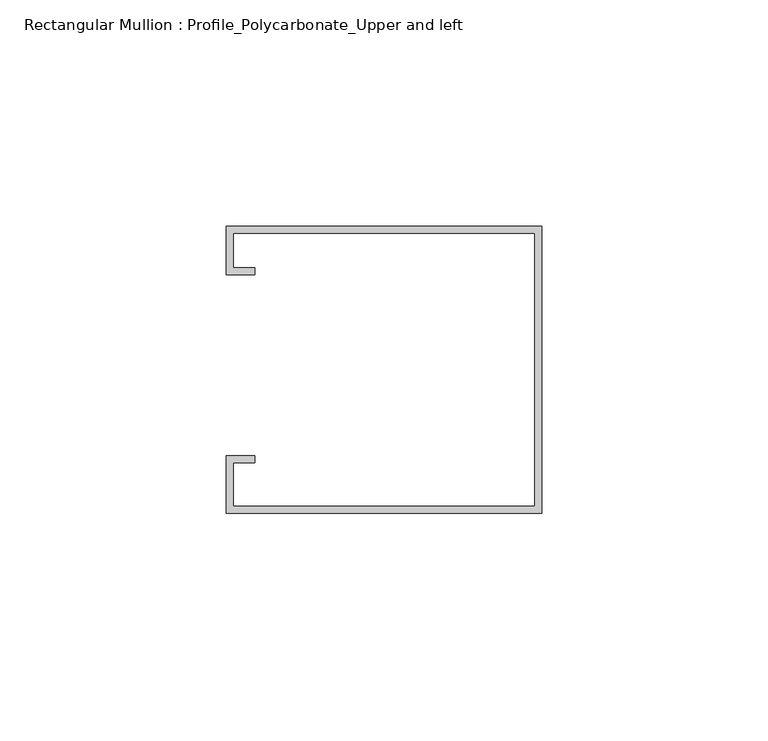
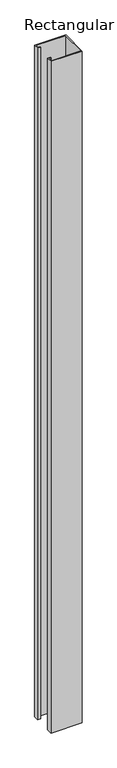
"""IFC4 building model written with IfcOpenShell, lengths in millimetres: member geometry, Rectangular Mullion : Profile_Polycarbonate_Upper and left."""

from ifc_helpers import new_model, si_unit, frame, origin, place, context, project, spatial, polyline, outline, extrude, source, transform, mapped, element, save


def rectangular_mullion_profile_polycarbonate_upper_and_left_256955de(model_context):
    return source(origin(), model_context, "Body", "SweptSolid", [
        extrude(outline(polyline([(0.0, -32.7), (-69.85, -32.7), (-69.85, -20.0), (-63.5, -20.0), (-63.5, -21.5875), (-68.2625, -21.5875), (-68.2625, -31.1125), (-1.5875, -31.1125), (-1.5875, 29.2125), (-68.2625, 29.2125), (-68.2625, 21.5875), (-63.5, 21.5875), (-63.5, 20.0), (-69.85, 20.0), (-69.85, 30.8), (0.0, 30.8), (0.0, -32.7)])), frame((0.0, 0.0, -1593.0298024), z_axis=(0.0, 0.0, 1.0), x_axis=(1.0, 0.0, 0.0)), (0.0, 0.0, 1.0), 1593.0298024),
    ])


if __name__ == "__main__":
    model = new_model("IFC4")
    model_context = context("Model", 3, world=origin())
    ifc_project = project(units=[si_unit("LENGTHUNIT", "METRE", prefix="MILLI")], contexts=[model_context])
    site = spatial("IfcSite", under=ifc_project)
    building = spatial("IfcBuilding", under=site)
    placement = place(None, origin())
    rectangular_mullion_profile_polycarbonate_upper_and_left_shape = rectangular_mullion_profile_polycarbonate_upper_and_left_256955de(model_context)
    element("IfcMember", 1, ObjectType="Rectangular Mullion : Profile_Polycarbonate_Upper and left", at=placement, inside=building, context=model_context, shape_type="MappedRepresentation", body=[
        mapped(rectangular_mullion_profile_polycarbonate_upper_and_left_shape, transform((0.0, 0.0, 0.0), x_axis=(1.0, 0.0, 0.0), y_axis=(0.0, 1.0, 0.0), z_axis=(0.0, 0.0, 1.0))),
    ])
    save(model, "model.ifc")

# Revit data of these elements
# Type "Rectangular Mullion : Profile_Polycarbonate_Upper and left"
#   built-in parameter 1007322 = 0.208333 (stored number, unit not read)
#   built-in parameter 1007321 = 0.00520833 (stored number, unit not read)
#   built-in parameter 1007320 = 0 (stored number, unit not read)
